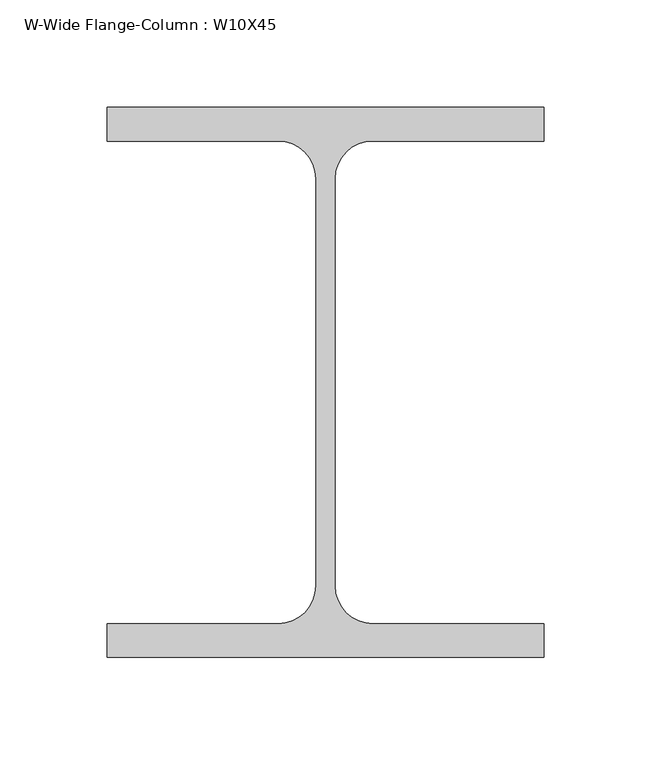
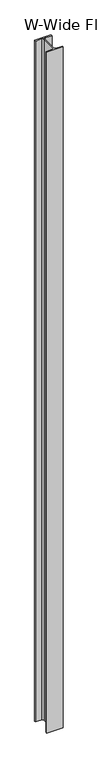
"""IFC4 building model written with IfcOpenShell, lengths in millimetres: column geometry, W-Wide Flange-Column : W10X45."""

from ifc_helpers import new_model, si_unit, point, frame, frame_2d, origin, place, context, project, spatial, polyline, circle_curve, trimmed, segment, composite_curve, outline, extrude, source, transform, mapped, element, save


def w_wide_flange_column_w10x45_18ccb682(model_context):
    return source(origin(), model_context, "Body", "SweptSolid", [
        extrude(outline(composite_curve([segment(polyline([(101.854, 128.27), (101.854, 112.522), (22.0345, 112.522)]), True, "CONTINUOUS"), segment(trimmed(circle_curve(frame_2d((22.0345, 94.9325)), 17.5895), [point((22.0345, 112.522))], [point((4.445, 94.9325))], True, "CARTESIAN"), True, "CONTINUOUS"), segment(polyline([(4.445, 94.9325), (4.445, -94.9325)]), True, "CONTINUOUS"), segment(trimmed(circle_curve(frame_2d((22.0345, -94.9325)), 17.5895), [point((4.445, -94.9325))], [point((22.0345, -112.522))], True, "CARTESIAN"), True, "CONTINUOUS"), segment(polyline([(22.0345, -112.522), (101.854, -112.522), (101.854, -128.27), (-101.854, -128.27), (-101.854, -112.522), (-22.0345, -112.522)]), True, "CONTINUOUS"), segment(trimmed(circle_curve(frame_2d((-22.0345, -94.9325)), 17.5895), [point((-22.0345, -112.522))], [point((-4.445, -94.9325))], True, "CARTESIAN"), True, "CONTINUOUS"), segment(polyline([(-4.445, -94.9325), (-4.445, 94.9325)]), True, "CONTINUOUS"), segment(trimmed(circle_curve(frame_2d((-22.0345, 94.9325)), 17.5895), [point((-4.445, 94.9325))], [point((-22.0345, 112.522))], True, "CARTESIAN"), True, "CONTINUOUS"), segment(polyline([(-22.0345, 112.522), (-101.854, 112.522), (-101.854, 128.27), (101.854, 128.27)]), True, "CONTINUOUS")], self_intersect=False)), frame((0.0, 0.0, 8756.65), z_axis=(0.0, 0.0, 1.0), x_axis=(1.0, 0.0, 0.0)), (0.0, 0.0, 1.0), 8870.95),
    ])


if __name__ == "__main__":
    model = new_model("IFC4")
    model_context = context("Model", 3, world=origin())
    ifc_project = project(units=[si_unit("LENGTHUNIT", "METRE", prefix="MILLI")], contexts=[model_context])
    site = spatial("IfcSite", under=ifc_project)
    building = spatial("IfcBuilding", under=site)
    placement = place(None, origin())
    w_wide_flange_column_w10x45_shape = w_wide_flange_column_w10x45_18ccb682(model_context)
    element("IfcColumn", 1, ObjectType="W-Wide Flange-Column : W10X45", at=placement, inside=building, context=model_context, shape_type="MappedRepresentation", body=[
        mapped(w_wide_flange_column_w10x45_shape, transform((0.0, 0.0, 0.0), x_axis=(1.0, 0.0, 0.0), y_axis=(0.0, 1.0, 0.0), z_axis=(0.0, 0.0, 1.0))),
    ])
    save(model, "model.ifc")

# Revit data of these elements
# Type "W-Wide Flange-Column : W10X45"
#   Assembly Code = "B10"
#   W = 45
#   bf = 0' - 8.02"
#   d = 0' - 10.1"
#   k = 0' - 1 5/16"
#   kr = 0' - 0.6925"
#   tf = 0' - 0.62"
#   tw = 0' - 0.35"
#   A = 0.0923611 SF
#   Structural Material [instance default] = Steel ASTM A992
# Element 1 (IfcColumn, "W-Wide Flange-Column : W10X45")
#   Materials on its faces: "Steel ASTM A992"
# Materials
#   "Steel ASTM A992": class "Metal", colour RGB 199 199 199, transparency 0, Description = "Structural steel 50ksi", Cost = 0
